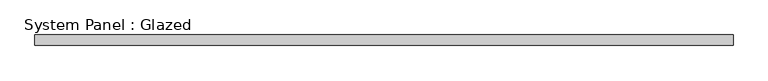
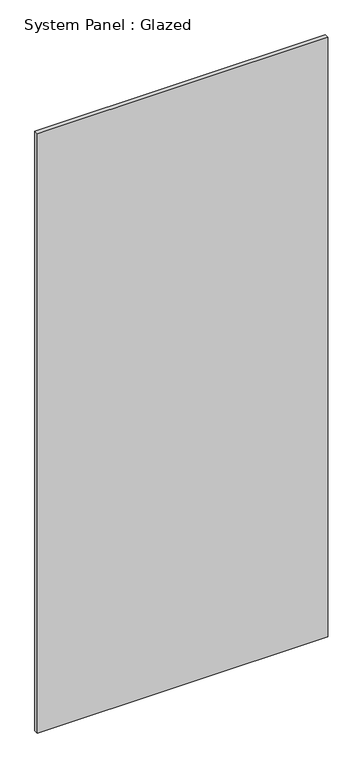
"""IFC4 building model written with IfcOpenShell, lengths in millimetres: plate geometry, System Panel : Glazed."""

import ifcopenshell
import ifcopenshell.guid

model = None  # the IFC model being written
_history = None  # IfcOwnerHistory: only IFC2X3 demands one
_inside = {}  # id of a spatial element -> (the spatial element, [elements in it])
_under = {}  # id of a project, library or spatial element -> (it, [spatial elements below it])
_declared = {}  # id of a project -> (the project, [libraries it declares])
_typed = {}  # id of a type object -> (the type object, [elements of that type])
_made_of = {}  # id of a material, layer set ... -> (it, [elements and type objects made of it])


def new_model(schema):
    """Start an empty IFC model of exactly this schema.

    Asked for "IFC4X3", IfcOpenShell would pick the latest addendum, in which some entities
    have other attributes; the version numbers below select the first issue.
    IFC2X3 requires an IfcOwnerHistory on every rooted entity: one is made here for all.
    """
    global model, _history
    if schema == "IFC4X3":
        model = ifcopenshell.file(schema_version=(4, 3, 0, 0))
    else:
        model = ifcopenshell.file(schema=schema)
    _inside.clear()
    _under.clear()
    _declared.clear()
    _typed.clear()
    _made_of.clear()
    _history = None
    if model.schema == "IFC2X3":
        org = make("IfcOrganization", Name="unknown")
        user = make(
            "IfcPersonAndOrganization",
            ThePerson=make("IfcPerson", FamilyName="unknown"),
            TheOrganization=org,
        )
        app = make(
            "IfcApplication",
            ApplicationDeveloper=org,
            Version="unknown",
            ApplicationFullName="unknown",
            ApplicationIdentifier="unknown",
        )
        _history = make(
            "IfcOwnerHistory",
            OwningUser=user,
            OwningApplication=app,
            ChangeAction="ADDED",
            CreationDate=0,
        )
    return model


def make(cls, **values):
    """One entity of the class cls with the attributes given. An attribute that is None is left unset."""
    return model.create_entity(
        cls, **{name: value for name, value in values.items() if value is not None}
    )


def rooted(cls, **values):
    """An entity with a GlobalId (a new one), such as an element, a storey or a relation."""
    return make(cls, GlobalId=ifcopenshell.guid.new(), OwnerHistory=_history, **values)


def si_unit(unit_type, name, prefix=None):
    """IfcSIUnit, for example si_unit("LENGTHUNIT", "METRE", prefix="MILLI")."""
    return make("IfcSIUnit", UnitType=unit_type, Prefix=prefix, Name=name)


def assignment(units):
    """IfcUnitAssignment: the units of a project."""
    return None if units is None else make("IfcUnitAssignment", Units=units)


def point(xyz):
    """IfcCartesianPoint."""
    return None if xyz is None else make("IfcCartesianPoint", Coordinates=xyz)


def direction(xyz):
    """IfcDirection."""
    return None if xyz is None else make("IfcDirection", DirectionRatios=xyz)


def frame(location, z_axis=None, x_axis=None):
    """IfcAxis2Placement3D, a coordinate frame: its origin and axes. An axis left out is left unset."""
    return make(
        "IfcAxis2Placement3D",
        Location=point(location),
        Axis=direction(z_axis),
        RefDirection=direction(x_axis),
    )


def origin():
    """The frame at (0, 0, 0) with its axes left unset."""
    return frame((0.0, 0.0, 0.0))


def origin_with_axes():
    """The frame at (0, 0, 0) with the z axis (0, 0, 1) and the x axis (1, 0, 0) written out."""
    return frame((0.0, 0.0, 0.0), z_axis=(0.0, 0.0, 1.0), x_axis=(1.0, 0.0, 0.0))


def place(relative_to, where):
    """IfcLocalPlacement: puts the frame where relative to a parent placement (None: the world)."""
    return make(
        "IfcLocalPlacement", PlacementRelTo=relative_to, RelativePlacement=where
    )


def context(
    kind, dimensions, precision=None, world=None, true_north=None, identifier=None
):
    """IfcGeometricRepresentationContext, for example the 3D "Model" context."""
    return make(
        "IfcGeometricRepresentationContext",
        ContextIdentifier=identifier,
        ContextType=kind,
        CoordinateSpaceDimension=dimensions,
        Precision=precision,
        WorldCoordinateSystem=world,
        TrueNorth=true_north,
    )


def project(units=None, contexts=None):
    """IfcProject with its units and contexts."""
    return rooted(
        "IfcProject",
        Name="project",
        RepresentationContexts=contexts,
        UnitsInContext=assignment(units),
    )


def spatial(cls, under=None, at=None, **own):
    """A site, building, storey or space (cls), placed at a placement, below another one or the project."""
    s = rooted(cls, ObjectPlacement=at, **own)
    if under is not None:
        _under.setdefault(under.id(), (under, []))[1].append(s)
    return s


def polyline(points):
    """IfcPolyline through the points."""
    return make("IfcPolyline", Points=[point(p) for p in points])


def outline(outer, holes=None, kind="AREA"):
    """IfcArbitraryClosedProfileDef: a profile drawn as a closed curve; with holes, ...WithVoids."""
    if holes is None:
        return make("IfcArbitraryClosedProfileDef", ProfileType=kind, OuterCurve=outer)
    return make(
        "IfcArbitraryProfileDefWithVoids",
        ProfileType=kind,
        OuterCurve=outer,
        InnerCurves=holes,
    )


def extrude(swept, where, along, depth):
    """IfcExtrudedAreaSolid: the profile swept, set in the frame where, extruded along a direction by depth."""
    return make(
        "IfcExtrudedAreaSolid",
        SweptArea=swept,
        Position=where,
        ExtrudedDirection=direction(along),
        Depth=depth,
    )


def shape(context_of_items, identifier, shape_type, items):
    """IfcShapeRepresentation: the items that make up one representation, for example the "Body"."""
    return make(
        "IfcShapeRepresentation",
        ContextOfItems=context_of_items,
        RepresentationIdentifier=identifier,
        RepresentationType=shape_type,
        Items=items,
    )


def source(mapping_origin, context_of_items, identifier, shape_type, items):
    """IfcRepresentationMap: a shape defined once, which mapped items show again and again."""
    return make(
        "IfcRepresentationMap",
        MappingOrigin=mapping_origin,
        MappedRepresentation=shape(context_of_items, identifier, shape_type, items),
    )


def transform(
    local_origin,
    x_axis=None,
    y_axis=None,
    z_axis=None,
    scale=None,
    scale2=None,
    scale3=None,
    uniform=True,
):
    """IfcCartesianTransformationOperator3D, or its non-uniform kind. x_axis, y_axis, z_axis: its Axis1, 2, 3."""
    if uniform:
        return make(
            "IfcCartesianTransformationOperator3D",
            Axis1=direction(x_axis),
            Axis2=direction(y_axis),
            LocalOrigin=point(local_origin),
            Scale=scale,
            Axis3=direction(z_axis),
        )
    return make(
        "IfcCartesianTransformationOperator3DnonUniform",
        Axis1=direction(x_axis),
        Axis2=direction(y_axis),
        LocalOrigin=point(local_origin),
        Scale=scale,
        Axis3=direction(z_axis),
        Scale2=scale2,
        Scale3=scale3,
    )


def mapped(mapping_source, mapping_target):
    """IfcMappedItem: shows the shape of a source again, moved by a transform."""
    return make(
        "IfcMappedItem", MappingSource=mapping_source, MappingTarget=mapping_target
    )


def made_of(thing, what):
    """Note that an element or type object is made of a material, layer set ...; save() writes the relation."""
    if what is not None:
        _made_of.setdefault(what.id(), (what, []))[1].append(thing)
    return thing


def element(
    cls,
    number,
    at=None,
    inside=None,
    cuts=None,
    type_object=None,
    material=None,
    context=None,
    identifier="Body",
    shape_type=None,
    held_by="IfcProductDefinitionShape",
    body=None,
    shapes=None,
    **own,
):
    """One element of the class cls, such as IfcWall. Its Tag is "e" and its number.

    at: its placement. inside: the storey or other place that contains it. cuts: it is an
    opening in that element (IfcRelVoidsElement). A single representation is given by context,
    identifier, shape_type and body (its items); several are given by shapes. held_by: the class
    of the entity that holds the representations. save() writes the other relations.
    """
    e = rooted(cls, Tag="e%d" % number, ObjectPlacement=at, **own)
    if body is not None:
        shapes = [shape(context, identifier, shape_type, body)]
    if shapes is not None:
        e.Representation = make(held_by, Representations=shapes)
    if inside is not None:
        _inside.setdefault(inside.id(), (inside, []))[1].append(e)
    if cuts is not None:
        rooted(
            "IfcRelVoidsElement", RelatingBuildingElement=cuts, RelatedOpeningElement=e
        )
    if type_object is not None:
        _typed.setdefault(type_object.id(), (type_object, []))[1].append(e)
    return made_of(e, material)


def aggregate(whole, parts):
    """IfcRelAggregates: a whole, such as a stair, and the parts it consists of."""
    return rooted("IfcRelAggregates", RelatingObject=whole, RelatedObjects=parts)


def save(model, path):
    """Write the relations noted so far, then the file.

    IfcRelAggregates (storeys below a building ...), IfcRelContainedInSpatialStructure (elements
    in a storey), IfcRelDefinesByType, IfcRelAssociatesMaterial and IfcRelDeclares: one each for
    every whole, place, type object, material and project.
    """
    for whole, parts in _under.values():
        aggregate(whole, parts)
    for where, things in _inside.values():
        rooted(
            "IfcRelContainedInSpatialStructure",
            RelatedElements=things,
            RelatingStructure=where,
        )
    for kind, things in _typed.values():
        rooted("IfcRelDefinesByType", RelatedObjects=things, RelatingType=kind)
    for what, things in _made_of.values():
        rooted("IfcRelAssociatesMaterial", RelatedObjects=things, RelatingMaterial=what)
    for by, libraries in _declared.values():
        rooted("IfcRelDeclares", RelatingContext=by, RelatedDefinitions=libraries)
    model.write(path)


def system_panel_glazed_2e91cb65(model_context):
    return source(origin(), model_context, "Body", "SweptSolid", [
        extrude(outline(polyline([(838.2000002, -44.45), (-838.2000002, -44.45), (-838.2000002, -19.05), (838.2000002, -19.05), (838.2000002, -44.45)])), origin_with_axes(), (0.0, 0.0, 1.0), 3657.6),
    ])


if __name__ == "__main__":
    model = new_model("IFC4")
    model_context = context("Model", 3, world=origin())
    ifc_project = project(units=[si_unit("LENGTHUNIT", "METRE", prefix="MILLI")], contexts=[model_context])
    site = spatial("IfcSite", under=ifc_project)
    building = spatial("IfcBuilding", under=site)
    placement = place(None, origin())
    system_panel_glazed_shape = system_panel_glazed_2e91cb65(model_context)
    element("IfcPlate", 1, ObjectType="System Panel : Glazed", at=placement, inside=building, context=model_context, shape_type="MappedRepresentation", body=[
        mapped(system_panel_glazed_shape, transform((0.0, 0.0, 0.0), x_axis=(1.0, 0.0, 0.0), y_axis=(0.0, 1.0, 0.0), z_axis=(0.0, 0.0, 1.0))),
    ])
    save(model, "model.ifc")

# Revit data of these elements
# Type "System Panel : Glazed"
#   Construction Type Id = "GSP4R"
#   Analytic Construction = "1/8 in Pilkington single glazing"
#   Visual Light Transmittance = 0.9
#   Solar Heat Gain Coefficient = 0.86
#   Heat Transfer Coefficient (U) = 1.18115 BTU/(h·ft²·°F)
#   Define Thermal Properties by = 1
# Element 1 (IfcPlate, "System Panel : Glazed")
#   Materials on its faces: "Glass"
# Materials
#   "Glass": class "Glass", colour RGB 0 128 192, transparency 0.75, Description = "Soda Lime Glass", Cost = 0
